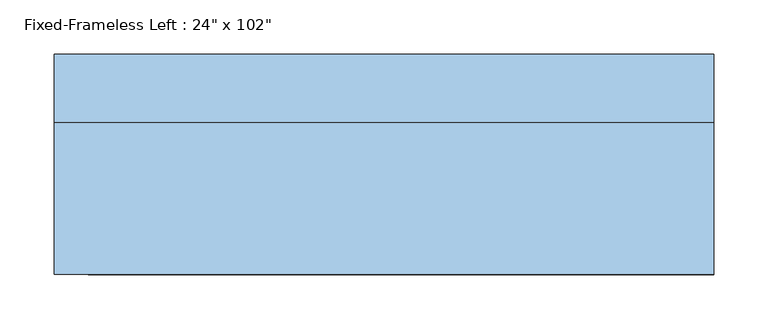
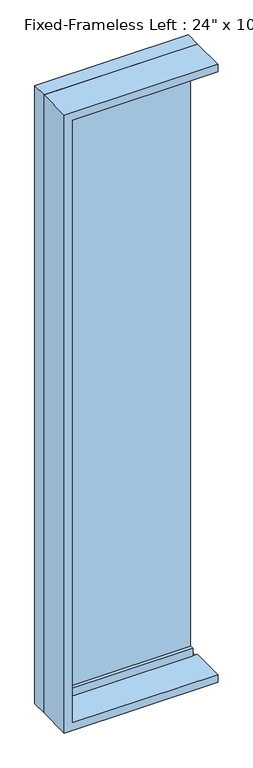
"""IFC4 building model written with IfcOpenShell, lengths in millimetres: window geometry."""

import ifcopenshell
import ifcopenshell.guid

model = None  # the IFC model being written
_history = None  # IfcOwnerHistory: only IFC2X3 demands one
_inside = {}  # id of a spatial element -> (the spatial element, [elements in it])
_under = {}  # id of a project, library or spatial element -> (it, [spatial elements below it])
_declared = {}  # id of a project -> (the project, [libraries it declares])
_typed = {}  # id of a type object -> (the type object, [elements of that type])
_made_of = {}  # id of a material, layer set ... -> (it, [elements and type objects made of it])


def new_model(schema):
    """Start an empty IFC model of exactly this schema.

    Asked for "IFC4X3", IfcOpenShell would pick the latest addendum, in which some entities
    have other attributes; the version numbers below select the first issue.
    IFC2X3 requires an IfcOwnerHistory on every rooted entity: one is made here for all.
    """
    global model, _history
    if schema == "IFC4X3":
        model = ifcopenshell.file(schema_version=(4, 3, 0, 0))
    else:
        model = ifcopenshell.file(schema=schema)
    _inside.clear()
    _under.clear()
    _declared.clear()
    _typed.clear()
    _made_of.clear()
    _history = None
    if model.schema == "IFC2X3":
        org = make("IfcOrganization", Name="unknown")
        user = make(
            "IfcPersonAndOrganization",
            ThePerson=make("IfcPerson", FamilyName="unknown"),
            TheOrganization=org,
        )
        app = make(
            "IfcApplication",
            ApplicationDeveloper=org,
            Version="unknown",
            ApplicationFullName="unknown",
            ApplicationIdentifier="unknown",
        )
        _history = make(
            "IfcOwnerHistory",
            OwningUser=user,
            OwningApplication=app,
            ChangeAction="ADDED",
            CreationDate=0,
        )
    return model


def make(cls, **values):
    """One entity of the class cls with the attributes given. An attribute that is None is left unset."""
    return model.create_entity(
        cls, **{name: value for name, value in values.items() if value is not None}
    )


def rooted(cls, **values):
    """An entity with a GlobalId (a new one), such as an element, a storey or a relation."""
    return make(cls, GlobalId=ifcopenshell.guid.new(), OwnerHistory=_history, **values)


def si_unit(unit_type, name, prefix=None):
    """IfcSIUnit, for example si_unit("LENGTHUNIT", "METRE", prefix="MILLI")."""
    return make("IfcSIUnit", UnitType=unit_type, Prefix=prefix, Name=name)


def assignment(units):
    """IfcUnitAssignment: the units of a project."""
    return None if units is None else make("IfcUnitAssignment", Units=units)


def point(xyz):
    """IfcCartesianPoint."""
    return None if xyz is None else make("IfcCartesianPoint", Coordinates=xyz)


def direction(xyz):
    """IfcDirection."""
    return None if xyz is None else make("IfcDirection", DirectionRatios=xyz)


def frame(location, z_axis=None, x_axis=None):
    """IfcAxis2Placement3D, a coordinate frame: its origin and axes. An axis left out is left unset."""
    return make(
        "IfcAxis2Placement3D",
        Location=point(location),
        Axis=direction(z_axis),
        RefDirection=direction(x_axis),
    )


def origin():
    """The frame at (0, 0, 0) with its axes left unset."""
    return frame((0.0, 0.0, 0.0))


def place(relative_to, where):
    """IfcLocalPlacement: puts the frame where relative to a parent placement (None: the world)."""
    return make(
        "IfcLocalPlacement", PlacementRelTo=relative_to, RelativePlacement=where
    )


def context(
    kind, dimensions, precision=None, world=None, true_north=None, identifier=None
):
    """IfcGeometricRepresentationContext, for example the 3D "Model" context."""
    return make(
        "IfcGeometricRepresentationContext",
        ContextIdentifier=identifier,
        ContextType=kind,
        CoordinateSpaceDimension=dimensions,
        Precision=precision,
        WorldCoordinateSystem=world,
        TrueNorth=true_north,
    )


def project(units=None, contexts=None):
    """IfcProject with its units and contexts."""
    return rooted(
        "IfcProject",
        Name="project",
        RepresentationContexts=contexts,
        UnitsInContext=assignment(units),
    )


def spatial(cls, under=None, at=None, **own):
    """A site, building, storey or space (cls), placed at a placement, below another one or the project."""
    s = rooted(cls, ObjectPlacement=at, **own)
    if under is not None:
        _under.setdefault(under.id(), (under, []))[1].append(s)
    return s


def polyline(points):
    """IfcPolyline through the points."""
    return make("IfcPolyline", Points=[point(p) for p in points])


def outline(outer, holes=None, kind="AREA"):
    """IfcArbitraryClosedProfileDef: a profile drawn as a closed curve; with holes, ...WithVoids."""
    if holes is None:
        return make("IfcArbitraryClosedProfileDef", ProfileType=kind, OuterCurve=outer)
    return make(
        "IfcArbitraryProfileDefWithVoids",
        ProfileType=kind,
        OuterCurve=outer,
        InnerCurves=holes,
    )


def extrude(swept, where, along, depth):
    """IfcExtrudedAreaSolid: the profile swept, set in the frame where, extruded along a direction by depth."""
    return make(
        "IfcExtrudedAreaSolid",
        SweptArea=swept,
        Position=where,
        ExtrudedDirection=direction(along),
        Depth=depth,
    )


def shape(context_of_items, identifier, shape_type, items):
    """IfcShapeRepresentation: the items that make up one representation, for example the "Body"."""
    return make(
        "IfcShapeRepresentation",
        ContextOfItems=context_of_items,
        RepresentationIdentifier=identifier,
        RepresentationType=shape_type,
        Items=items,
    )


def source(mapping_origin, context_of_items, identifier, shape_type, items):
    """IfcRepresentationMap: a shape defined once, which mapped items show again and again."""
    return make(
        "IfcRepresentationMap",
        MappingOrigin=mapping_origin,
        MappedRepresentation=shape(context_of_items, identifier, shape_type, items),
    )


def transform(
    local_origin,
    x_axis=None,
    y_axis=None,
    z_axis=None,
    scale=None,
    scale2=None,
    scale3=None,
    uniform=True,
):
    """IfcCartesianTransformationOperator3D, or its non-uniform kind. x_axis, y_axis, z_axis: its Axis1, 2, 3."""
    if uniform:
        return make(
            "IfcCartesianTransformationOperator3D",
            Axis1=direction(x_axis),
            Axis2=direction(y_axis),
            LocalOrigin=point(local_origin),
            Scale=scale,
            Axis3=direction(z_axis),
        )
    return make(
        "IfcCartesianTransformationOperator3DnonUniform",
        Axis1=direction(x_axis),
        Axis2=direction(y_axis),
        LocalOrigin=point(local_origin),
        Scale=scale,
        Axis3=direction(z_axis),
        Scale2=scale2,
        Scale3=scale3,
    )


def mapped(mapping_source, mapping_target):
    """IfcMappedItem: shows the shape of a source again, moved by a transform."""
    return make(
        "IfcMappedItem", MappingSource=mapping_source, MappingTarget=mapping_target
    )


def made_of(thing, what):
    """Note that an element or type object is made of a material, layer set ...; save() writes the relation."""
    if what is not None:
        _made_of.setdefault(what.id(), (what, []))[1].append(thing)
    return thing


def element(
    cls,
    number,
    at=None,
    inside=None,
    cuts=None,
    type_object=None,
    material=None,
    context=None,
    identifier="Body",
    shape_type=None,
    held_by="IfcProductDefinitionShape",
    body=None,
    shapes=None,
    **own,
):
    """One element of the class cls, such as IfcWall. Its Tag is "e" and its number.

    at: its placement. inside: the storey or other place that contains it. cuts: it is an
    opening in that element (IfcRelVoidsElement). A single representation is given by context,
    identifier, shape_type and body (its items); several are given by shapes. held_by: the class
    of the entity that holds the representations. save() writes the other relations.
    """
    e = rooted(cls, Tag="e%d" % number, ObjectPlacement=at, **own)
    if body is not None:
        shapes = [shape(context, identifier, shape_type, body)]
    if shapes is not None:
        e.Representation = make(held_by, Representations=shapes)
    if inside is not None:
        _inside.setdefault(inside.id(), (inside, []))[1].append(e)
    if cuts is not None:
        rooted(
            "IfcRelVoidsElement", RelatingBuildingElement=cuts, RelatedOpeningElement=e
        )
    if type_object is not None:
        _typed.setdefault(type_object.id(), (type_object, []))[1].append(e)
    return made_of(e, material)


def aggregate(whole, parts):
    """IfcRelAggregates: a whole, such as a stair, and the parts it consists of."""
    return rooted("IfcRelAggregates", RelatingObject=whole, RelatedObjects=parts)


def save(model, path):
    """Write the relations noted so far, then the file.

    IfcRelAggregates (storeys below a building ...), IfcRelContainedInSpatialStructure (elements
    in a storey), IfcRelDefinesByType, IfcRelAssociatesMaterial and IfcRelDeclares: one each for
    every whole, place, type object, material and project.
    """
    for whole, parts in _under.values():
        aggregate(whole, parts)
    for where, things in _inside.values():
        rooted(
            "IfcRelContainedInSpatialStructure",
            RelatedElements=things,
            RelatingStructure=where,
        )
    for kind, things in _typed.values():
        rooted("IfcRelDefinesByType", RelatedObjects=things, RelatingType=kind)
    for what, things in _made_of.values():
        rooted("IfcRelAssociatesMaterial", RelatedObjects=things, RelatingMaterial=what)
    for by, libraries in _declared.values():
        rooted("IfcRelDeclares", RelatingContext=by, RelatedDefinitions=libraries)
    model.write(path)


def window_40525b03(model_context):
    return source(origin(), model_context, "Body", "SweptSolid", [
        extrude(outline(polyline([(247.65, 53.975), (-279.4, 53.975), (-279.4, 66.675), (247.65, 66.675), (247.65, 53.975)])), frame((0.0, 0.0, 368.3), z_axis=(0.0, 0.0, 1.0), x_axis=(1.0, 0.0, 0.0)), (0.0, 0.0, 1.0), 2463.8),
        extrude(outline(polyline([(2876.55, -323.85), (323.85, -323.85), (323.85, 247.65), (368.3, 247.65), (368.3, -279.4), (2832.1, -279.4), (2832.1, 247.65), (2876.55, 247.65), (2876.55, -323.85)])), frame((0.0, 38.1, 0.0), z_axis=(0.0, 1.0, 0.0), x_axis=(0.0, 0.0, 1.0)), (0.0, 0.0, 1.0), 44.45),
        extrude(outline(polyline([(2895.6, -342.9), (304.8, -342.9), (304.8, 266.7), (336.55, 266.7), (336.55, -311.15), (2863.85, -311.15), (2863.85, 266.7), (2895.6, 266.7), (2895.6, -342.9)])), frame((0.0, -101.6, 0.0), z_axis=(0.0, 1.0, 0.0), x_axis=(0.0, 0.0, 1.0)), (0.0, 0.0, 1.0), 139.7),
        extrude(outline(polyline([(2895.6, 266.7), (2895.6, -342.9), (304.8, -342.9), (304.8, 266.7), (323.85, 266.7), (323.85, -323.85), (2876.55, -323.85), (2876.55, 266.7), (2895.6, 266.7)])), frame((0.0, 38.1, 0.0), z_axis=(0.0, 1.0, 0.0), x_axis=(0.0, 0.0, 1.0)), (0.0, 0.0, 1.0), 63.5),
    ])


if __name__ == "__main__":
    model = new_model("IFC4")
    model_context = context("Model", 3, world=origin())
    ifc_project = project(units=[si_unit("LENGTHUNIT", "METRE", prefix="MILLI")], contexts=[model_context])
    site = spatial("IfcSite", under=ifc_project)
    building = spatial("IfcBuilding", under=site)
    placement = place(None, origin())
    window_shape = window_40525b03(model_context)
    element("IfcWindow", 1, ObjectType="Fixed-Frameless Left : 24\" x 102\"", at=placement, inside=building, context=model_context, shape_type="MappedRepresentation", body=[
        mapped(window_shape, transform((0.0, 0.0, 0.0), x_axis=(1.0, 0.0, 0.0), y_axis=(0.0, 1.0, 0.0), z_axis=(0.0, 0.0, 1.0))),
    ])
    save(model, "model.ifc")

# Revit data of these elements
# Type "Fixed-Frameless Left : 24\" x 102\""
#   Type Mark = "72"
#   Assembly Code = "B2020100"
#   Height = 8' - 6"
#   Default Sill Height = 1' - 0"
#   Width = 2' - 0"
#   Window Inset = 0' - 0 3/4"
#   Glass Pane Material = Glass
#   Sash Material = Sash
#   Wall Closure = (empty or 0)
# Element 1 (IfcWindow, "Fixed-Frameless Left : 24\" x 102\"")
#   Materials on its faces: "Sash", "Glass"
# Materials
#   "Glass": class "Glass", colour RGB 0 128 192, transparency 0.75
#   "Sash": class "Wood", colour RGB 224 178 126, transparency 0
